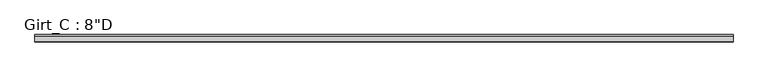
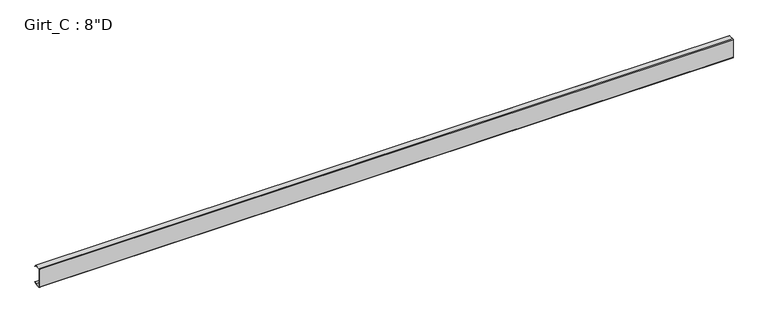
"""IFC4 building model written with IfcOpenShell, lengths in millimetres: beam geometry."""

from ifc_helpers import new_model, si_unit, point, frame, frame_2d, origin, place, context, project, spatial, polyline, circle_curve, trimmed, segment, composite_curve, outline, extrude, source, transform, mapped, element, save


def beam_e8be4c3a(model_context):
    return source(origin(), model_context, "Body", "SweptSolid", [
        extrude(outline(composite_curve([segment(polyline([(63.5, 101.6), (75.745104, 87.0068534), (73.6169367, 85.221109), (62.204539, 98.821875), (3.3005807, 98.821875)]), True, "CONTINUOUS"), segment(trimmed(circle_curve(frame_2d((3.3741066, 96.8381931)), 1.9850441), [point((3.3005807, 98.821875))], [point((1.3890625, 96.8381931))], True, "CARTESIAN"), True, "CONTINUOUS"), segment(polyline([(1.3890625, 96.8381931), (1.3890625, -96.8389339)]), True, "CONTINUOUS"), segment(trimmed(circle_curve(frame_2d((3.3748024, -96.8389339)), 1.9857399), [point((1.3890625, -96.8389339))], [point((3.2694106, -98.821875))], True, "CARTESIAN"), True, "CONTINUOUS"), segment(polyline([(3.2694106, -98.821875), (62.204539, -98.821875), (73.6169367, -85.221109), (75.745104, -87.0068534), (63.5, -101.6), (3.3734375, -101.6)]), True, "CONTINUOUS"), segment(trimmed(circle_curve(frame_2d((3.3734375, -96.8375)), 4.7625), [point((3.3734375, -101.6))], [point((-1.3890625, -96.8375))], False, "CARTESIAN"), True, "CONTINUOUS"), segment(polyline([(-1.3890625, -96.8375), (-1.3890625, 96.8375)]), True, "CONTINUOUS"), segment(trimmed(circle_curve(frame_2d((3.3734375, 96.8375)), 4.7625), [point((-1.3890625, 96.8375))], [point((3.3734375, 101.6))], False, "CARTESIAN"), True, "CONTINUOUS"), segment(polyline([(3.3734375, 101.6), (63.5, 101.6)]), True, "CONTINUOUS")], self_intersect=False)), frame((-3692.525, 0.0, 0.0), z_axis=(1.0, 0.0, 0.0), x_axis=(0.0, 1.0, 0.0)), (0.0, 0.0, 1.0), 7159.625),
    ])


if __name__ == "__main__":
    model = new_model("IFC4")
    model_context = context("Model", 3, world=origin())
    ifc_project = project(units=[si_unit("LENGTHUNIT", "METRE", prefix="MILLI")], contexts=[model_context])
    site = spatial("IfcSite", under=ifc_project)
    building = spatial("IfcBuilding", under=site)
    placement = place(None, origin())
    beam_shape = beam_e8be4c3a(model_context)
    element("IfcBeam", 1, ObjectType="Girt_C : 8\"D", at=placement, inside=building, context=model_context, shape_type="MappedRepresentation", body=[
        mapped(beam_shape, transform((0.0, 0.0, 0.0), x_axis=(1.0, 0.0, 0.0), y_axis=(0.0, 1.0, 0.0), z_axis=(0.0, 0.0, 1.0))),
    ])
    save(model, "model.ifc")

# Revit data of these elements
# Type "Girt_C : 8\"D"
#   Web_Thickness = 0' - 0 7/64"
#   Length [instance default] = 10' - 0"
#   Leg_1 = 0' - 2 1/2"
#   Height = 0' - 8"
#   Structural Material [instance default] = none
# Element 1 (IfcBeam, "Girt_C : 8\"D")
#   Structural Material = Steel
#   Materials on its faces: "Steel"
# Materials
#   "Steel": class "Metal", colour RGB 118 118 114, transparency 0, Description = "Steel, mill finish", Cost = 0
